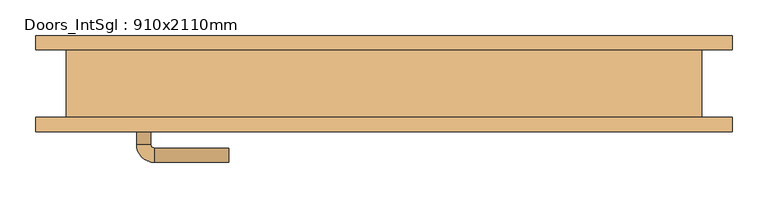
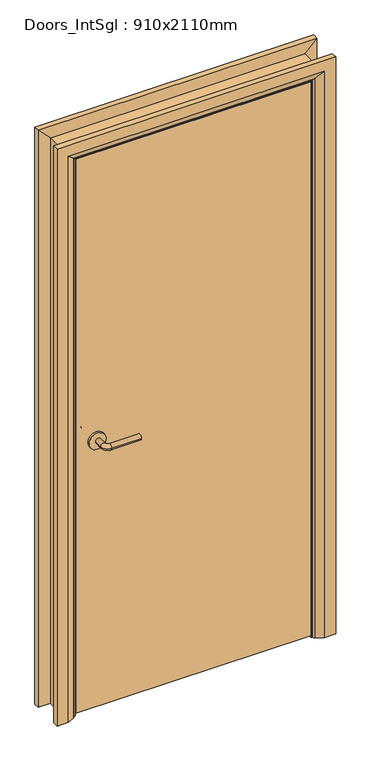
"""IFC4 building model written with IfcOpenShell, lengths in millimetres: door geometry, Doors_IntSgl : 910x2110mm."""

from ifc_helpers import new_model, si_unit, point, frame, frame_2d, origin, place, context, project, spatial, polyline, circle_curve, ellipse_curve, trimmed, segment, composite_curve, outline, extrude, faceted_brep, source, transform, mapped, element, save
from ifc_brep_helpers import plane_surface, cylinder_surface, revolved_surface, advanced_brep


def doors_intsgl_910x2110mm_17b3a64a(model_context):
    return source(origin(), model_context, "Body", "SolidModel", [
        advanced_brep(
        [(-348.0, -1.5, 1000.0), (-328.0, -1.5, 1000.0), (-348.0, 28.5, 1000.0), (-328.0, 28.5, 1000.0), (-323.0, 33.5, 1000.0), (-323.0, 53.5, 1000.0), (-218.0, 53.5, 1000.0), (-218.0, 33.5, 1000.0)],
        [
            (0, 1, circle_curve(frame((-338.0, -1.5, 1000.0), z_axis=(0.0, -1.0, 0.0), x_axis=(1.0, 0.0, 0.0)), 10.0)),
            (1, 0, circle_curve(frame((-338.0, -1.5, 1000.0), z_axis=(0.0, -1.0, 0.0), x_axis=(1.0, 0.0, 0.0)), 10.0)),
            (0, 2),
            (2, 3, circle_curve(frame((-338.0, 28.5, 1000.0), z_axis=(0.0, -1.0, 0.0), x_axis=(1.0, 0.0, 0.0)), 10.0)),
            (3, 1),
            (3, 2, circle_curve(frame((-338.0, 28.5, 1000.0), z_axis=(0.0, -1.0, 0.0), x_axis=(1.0, 0.0, 0.0)), 10.0)),
            (4, 3, circle_curve(frame((-323.0, 28.5, 1000.0), z_axis=(0.0, 0.0, 1.0), x_axis=(-1.0, 0.0, 0.0)), 5.0)),
            (2, 5, circle_curve(frame((-323.0, 28.5, 1000.0), z_axis=(0.0, 0.0, -1.0), x_axis=(-1.0, 0.0, 0.0)), 25.0)),
            (5, 4, circle_curve(frame((-323.0, 43.5, 1000.0), z_axis=(-1.0, 0.0, 0.0), x_axis=(0.0, -1.0, 0.0)), 10.0)),
            (4, 5, circle_curve(frame((-323.0, 43.5, 1000.0), z_axis=(-1.0, 0.0, 0.0), x_axis=(0.0, -1.0, 0.0)), 10.0)),
            (6, 7, circle_curve(frame((-218.0, 43.5, 1000.0), z_axis=(1.0, 0.0, 0.0), x_axis=(0.0, -1.0, 0.0)), 10.0)),
            (7, 6, circle_curve(frame((-218.0, 43.5, 1000.0), z_axis=(1.0, 0.0, 0.0), x_axis=(0.0, -1.0, 0.0)), 10.0)),
            (5, 6),
            (7, 4),
        ],
        [
            plane_surface(frame((-338.0, -1.5, 1000.0), z_axis=(0.0, -1.0, 0.0), x_axis=(0.0, 0.0, 1.0))),
            cylinder_surface(frame((-338.0, -1.5, 1000.0), z_axis=(0.0, -1.0, 0.0), x_axis=(1.0, 0.0, 0.0)), 10.0),
            revolved_surface(trimmed(ellipse_curve(frame((-338.0, 28.5, 1000.0), z_axis=(0.0, -1.0, 0.0), x_axis=(1.0, 0.0, 0.0)), 10.0, 10.0), [point((-348.0, 28.5, 1000.0))], [point((-328.0, 28.5, 1000.0))], True, "CARTESIAN"), (-323.0, 28.5, 1000.0), (0.0, 0.0, -1.0)),
            revolved_surface(trimmed(ellipse_curve(frame((-338.0, 28.5, 1000.0), z_axis=(0.0, -1.0, 0.0), x_axis=(1.0, 0.0, 0.0)), 10.0, 10.0), [point((-328.0, 28.5, 1000.0))], [point((-348.0, 28.5, 1000.0))], True, "CARTESIAN"), (-323.0, 28.5, 1000.0), (0.0, 0.0, -1.0)),
            plane_surface(frame((-218.0, 43.5, 1000.0), z_axis=(1.0, 0.0, 0.0), x_axis=(0.0, 0.0, 1.0))),
            cylinder_surface(frame((-323.0, 43.5, 1000.0), z_axis=(-1.0, 0.0, 0.0), x_axis=(0.0, -1.0, 0.0)), 10.0),
        ],
        [
            (0, [[1, 2]]),
            (1, [[-1, 3, 4, 5]]),
            (1, [[-2, -5, 6, -3]]),
            (2, [[7, -4, 8, 9]]),
            (3, [[-8, -6, -7, 10]]),
            (4, [[11, 12]]),
            (5, [[-9, 13, -12, 14]]),
            (5, [[-10, -14, -11, -13]]),
        ],
    ),
        extrude(outline(composite_curve([segment(trimmed(circle_curve(frame_2d((1000.0, -340.5)), 30.0), [point((1000.0, -370.5))], [point((1000.0, -310.5))], False, "CARTESIAN"), True, "CONTINUOUS"), segment(trimmed(circle_curve(frame_2d((1000.0, -340.5)), 30.0), [point((1000.0, -310.5))], [point((1000.0, -370.5))], False, "CARTESIAN"), True, "CONTINUOUS")], self_intersect=False)), frame((0.0, -9.5, 0.0), z_axis=(0.0, 1.0, 0.0), x_axis=(0.0, 0.0, 1.0)), (0.0, 0.0, 1.0), 8.0),
        advanced_brep(
        [(-348.0, -55.5, 1000.0), (-328.0, -55.5, 1000.0), (-328.0, -85.5, 1000.0), (-348.0, -85.5, 1000.0), (-323.0, -90.5, 1000.0), (-323.0, -110.5, 1000.0), (-218.0, -110.5, 1000.0), (-218.0, -90.5, 1000.0)],
        [
            (0, 1, circle_curve(frame((-338.0, -55.5, 1000.0), z_axis=(0.0, 1.0, 0.0), x_axis=(1.0, 0.0, 0.0)), 10.0)),
            (1, 0, circle_curve(frame((-338.0, -55.5, 1000.0), z_axis=(0.0, 1.0, 0.0), x_axis=(1.0, 0.0, 0.0)), 10.0)),
            (1, 2),
            (2, 3, circle_curve(frame((-338.0, -85.5, 1000.0), z_axis=(0.0, 1.0, 0.0), x_axis=(1.0, 0.0, 0.0)), 10.0)),
            (3, 0),
            (3, 2, circle_curve(frame((-338.0, -85.5, 1000.0), z_axis=(0.0, 1.0, 0.0), x_axis=(1.0, 0.0, 0.0)), 10.0)),
            (4, 5, circle_curve(frame((-323.0, -100.5, 1000.0), z_axis=(-1.0, 0.0, 0.0), x_axis=(0.0, 1.0, 0.0)), 10.0)),
            (5, 3, circle_curve(frame((-323.0, -85.5, 1000.0), z_axis=(0.0, 0.0, -1.0), x_axis=(-1.0, 0.0, 0.0)), 25.0)),
            (2, 4, circle_curve(frame((-323.0, -85.5, 1000.0), z_axis=(0.0, 0.0, 1.0), x_axis=(-1.0, 0.0, 0.0)), 5.0)),
            (5, 4, circle_curve(frame((-323.0, -100.5, 1000.0), z_axis=(-1.0, 0.0, 0.0), x_axis=(0.0, 1.0, 0.0)), 10.0)),
            (6, 7, circle_curve(frame((-218.0, -100.5, 1000.0), z_axis=(1.0, 0.0, 0.0), x_axis=(0.0, 1.0, 0.0)), 10.0)),
            (7, 6, circle_curve(frame((-218.0, -100.5, 1000.0), z_axis=(1.0, 0.0, 0.0), x_axis=(0.0, 1.0, 0.0)), 10.0)),
            (4, 7),
            (6, 5),
        ],
        [
            plane_surface(frame((-338.0, -55.5, 1000.0), z_axis=(0.0, 1.0, 0.0), x_axis=(0.0, 0.0, 1.0))),
            cylinder_surface(frame((-338.0, -55.5, 1000.0), z_axis=(0.0, 1.0, 0.0), x_axis=(1.0, 0.0, 0.0)), 10.0),
            revolved_surface(trimmed(ellipse_curve(frame((-338.0, -85.5, 1000.0), z_axis=(0.0, -1.0, 0.0), x_axis=(1.0, 0.0, 0.0)), 10.0, 10.0), [point((-348.0, -85.5, 1000.0))], [point((-328.0, -85.5, 1000.0))], True, "CARTESIAN"), (-323.0, -85.5, 1000.0), (0.0, 0.0, -1.0)),
            revolved_surface(trimmed(ellipse_curve(frame((-338.0, -85.5, 1000.0), z_axis=(0.0, -1.0, 0.0), x_axis=(1.0, 0.0, 0.0)), 10.0, 10.0), [point((-328.0, -85.5, 1000.0))], [point((-348.0, -85.5, 1000.0))], True, "CARTESIAN"), (-323.0, -85.5, 1000.0), (0.0, 0.0, -1.0)),
            plane_surface(frame((-218.0, -100.5, 1000.0), z_axis=(1.0, 0.0, 0.0), x_axis=(0.0, 0.0, 1.0))),
            cylinder_surface(frame((-323.0, -100.5, 1000.0), z_axis=(-1.0, 0.0, 0.0), x_axis=(0.0, 1.0, 0.0)), 10.0),
        ],
        [
            (0, [[1, 2]]),
            (1, [[3, 4, 5, -2]]),
            (1, [[-5, 6, -3, -1]]),
            (2, [[7, 8, -4, 9]]),
            (3, [[10, -9, -6, -8]]),
            (4, [[11, 12]]),
            (5, [[13, -11, 14, -7]]),
            (5, [[-14, -12, -13, -10]]),
        ],
    ),
        extrude(outline(composite_curve([segment(trimmed(circle_curve(frame_2d((1000.0, -340.5)), 30.0), [point((1000.0, -370.5))], [point((1000.0, -310.5))], False, "CARTESIAN"), True, "CONTINUOUS"), segment(trimmed(circle_curve(frame_2d((1000.0, -340.5)), 30.0), [point((1000.0, -310.5))], [point((1000.0, -370.5))], False, "CARTESIAN"), True, "CONTINUOUS")], self_intersect=False)), frame((0.0, -55.5, 0.0), z_axis=(0.0, 1.0, 0.0), x_axis=(0.0, 0.0, 1.0)), (0.0, 0.0, 1.0), 8.0),
        extrude(outline(polyline([(413.0, -9.5), (413.0, -47.5), (-413.0, -47.5), (-413.0, -9.5), (413.0, -9.5)])), frame((0.0, 0.0, 8.0), z_axis=(0.0, 0.0, 1.0), x_axis=(1.0, 0.0, 0.0)), (0.0, 0.0, 1.0), 2060.0),
        advanced_brep(
        [(490.0, -67.5, 0.0), (450.0, -67.5, 0.0), (424.0, -53.5, 0.0), (420.0, -47.5, 0.0), (490.0, -47.5, 0.0), (490.0, -47.5, 2145.0), (490.0, -67.5, 2145.0), (420.0, -47.5, 2075.0), (-420.0, -47.5, 2075.0), (-420.0, -47.5, 0.0), (-490.0, -47.5, 0.0), (-490.0, -47.5, 2145.0), (424.0, -53.5, 2079.0), (450.0, -67.5, 2105.0), (-490.0, -67.5, 2145.0), (-490.0, -67.5, 0.0), (-450.0, -67.5, 0.0), (-450.0, -67.5, 2105.0), (-424.0, -53.5, 2079.0), (-424.0, -53.5, 0.0)],
        [
            (0, 1),
            (1, 2),
            (2, 3, circle_curve(frame((428.0, -46.5, 0.0), z_axis=(0.0, 0.0, -1.0), x_axis=(1.0, 0.0, 0.0)), 8.0622577)),
            (3, 4),
            (4, 0),
            (4, 5),
            (5, 6),
            (6, 0),
            (3, 7),
            (7, 8),
            (8, 9),
            (9, 10),
            (10, 11),
            (11, 5),
            (2, 12),
            (12, 7, ellipse_curve(frame((428.0, -46.5, 2083.0), z_axis=(0.7071067811865475, 0.0, -0.7071067811865475), x_axis=(-0.7071067811865474, 0.0, -0.7071067811865476)), 11.4017543, 8.0622577)),
            (1, 13),
            (13, 12),
            (6, 14),
            (14, 15),
            (15, 16),
            (16, 17),
            (17, 13),
            (11, 14),
            (12, 18),
            (18, 8, ellipse_curve(frame((-428.0, -46.5, 2083.0), z_axis=(0.7071067811865475, 0.0, 0.7071067811865475), x_axis=(0.7071067811865476, 0.0, -0.7071067811865474)), 11.4017543, 8.0622577)),
            (17, 18),
            (15, 10),
            (9, 19, circle_curve(frame((-428.0, -46.5, 0.0), z_axis=(0.0, 0.0, -1.0), x_axis=(-1.0, 0.0, 0.0)), 8.0622577)),
            (19, 16),
            (18, 19),
        ],
        [
            plane_surface(frame((420.0, -47.5, 0.0), z_axis=(0.0, 0.0, -1.0), x_axis=(0.0, 1.0, 0.0))),
            plane_surface(frame((490.0, -67.5, 0.0), z_axis=(1.0, 0.0, 0.0), x_axis=(0.0, 0.0, 1.0))),
            plane_surface(frame((490.0, -47.5, 0.0), z_axis=(0.0, 1.0, 0.0), x_axis=(0.0, 0.0, 1.0))),
            cylinder_surface(frame((428.0, -46.5, 0.0), z_axis=(0.0, 0.0, -1.0), x_axis=(1.0, 0.0, 0.0)), 8.0622577),
            plane_surface(frame((424.0, -53.5, 0.0), z_axis=(-0.4740998230350126, -0.880471099922178, 0.0), x_axis=(0.0, 0.0, 1.0))),
            plane_surface(frame((450.0, -67.5, 0.0), z_axis=(0.0, -1.0, 0.0), x_axis=(0.0, 0.0, 1.0))),
            plane_surface(frame((490.0, -67.5, 2145.0), z_axis=(0.0, 0.0, 1.0), x_axis=(-1.0, 0.0, 0.0))),
            cylinder_surface(frame((420.0, -46.5, 2083.0), z_axis=(1.0, 0.0, 0.0), x_axis=(0.0, 0.0, 1.0)), 8.0622577),
            plane_surface(frame((424.0, -53.5, 2079.0), z_axis=(0.0, -0.8804710999221764, -0.4740998230350154), x_axis=(-1.0, 0.0, 0.0))),
            plane_surface(frame((-420.0, -47.5, 0.0), z_axis=(0.0, 0.0, -1.0), x_axis=(0.0, 1.0, 0.0))),
            plane_surface(frame((-490.0, -67.5, 2145.0), z_axis=(-1.0, 0.0, 0.0), x_axis=(0.0, 0.0, -1.0))),
            cylinder_surface(frame((-428.0, -46.5, 2075.0), z_axis=(0.0, 0.0, 1.0), x_axis=(-1.0, 0.0, 0.0)), 8.0622577),
            plane_surface(frame((-424.0, -53.5, 2079.0), z_axis=(0.47409982303501824, -0.8804710999221749, 0.0), x_axis=(0.0, 0.0, -1.0))),
        ],
        [
            (0, [[1, 2, 3, 4, 5]]),
            (1, [[6, 7, 8, -5]]),
            (2, [[9, 10, 11, 12, 13, 14, -6, -4]]),
            (3, [[15, 16, -9, -3]]),
            (4, [[17, 18, -15, -2]]),
            (5, [[-8, 19, 20, 21, 22, 23, -17, -1]]),
            (6, [[-14, 24, -19, -7]]),
            (7, [[25, 26, -10, -16]]),
            (8, [[-23, 27, -25, -18]]),
            (9, [[28, -12, 29, 30, -21]]),
            (10, [[-13, -28, -20, -24]]),
            (11, [[31, -29, -11, -26]]),
            (12, [[-22, -30, -31, -27]]),
        ],
    ),
        extrude(outline(polyline([(0.0, -396.0), (2051.0, -396.0), (2051.0, 396.0), (0.0, 396.0), (0.0, 415.0), (2070.0, 415.0), (2070.0, -415.0), (0.0, -415.0), (0.0, -396.0)])), frame((0.0, -7.5, 0.0), z_axis=(0.0, 1.0, 0.0), x_axis=(0.0, 0.0, 1.0)), (0.0, 0.0, 1.0), 32.0),
        advanced_brep(
        [(-490.0, 67.5, 0.0), (-450.0, 67.5, 0.0), (-424.0, 53.5, 0.0), (-420.0, 47.5, 0.0), (-490.0, 47.5, 0.0), (-490.0, 47.5, 2145.0), (-490.0, 67.5, 2145.0), (-420.0, 47.5, 2075.0), (-424.0, 53.5, 2079.0), (-450.0, 67.5, 2105.0), (490.0, 47.5, 2145.0), (490.0, 67.5, 2145.0), (420.0, 47.5, 2075.0), (424.0, 53.5, 2079.0), (450.0, 67.5, 2105.0), (490.0, 67.5, 0.0), (490.0, 47.5, 0.0), (420.0, 47.5, 0.0), (424.0, 53.5, 0.0), (450.0, 67.5, 0.0)],
        [
            (0, 1),
            (1, 2),
            (2, 3, circle_curve(frame((-428.0, 46.5, 0.0), z_axis=(0.0, 0.0, -1.0), x_axis=(-1.0, 0.0, 0.0)), 8.0622577)),
            (3, 4),
            (4, 0),
            (4, 5),
            (5, 6),
            (6, 0),
            (3, 7),
            (7, 5),
            (2, 8),
            (8, 7, ellipse_curve(frame((-428.0, 46.5, 2083.0), z_axis=(-0.7071067811865475, 0.0, -0.7071067811865475), x_axis=(0.7071067811865474, 0.0, -0.7071067811865476)), 11.4017543, 8.0622577)),
            (1, 9),
            (9, 8),
            (6, 9),
            (5, 10),
            (10, 11),
            (11, 6),
            (7, 12),
            (12, 10),
            (8, 13),
            (13, 12, ellipse_curve(frame((428.0, 46.5, 2083.0), z_axis=(-0.7071067811865475, 0.0, 0.7071067811865475), x_axis=(-0.7071067811865476, 0.0, -0.7071067811865474)), 11.4017543, 8.0622577)),
            (9, 14),
            (14, 13),
            (11, 14),
            (15, 16),
            (16, 17),
            (17, 18, circle_curve(frame((428.0, 46.5, 0.0), z_axis=(0.0, 0.0, -1.0), x_axis=(1.0, 0.0, 0.0)), 8.0622577)),
            (18, 19),
            (19, 15),
            (10, 16),
            (15, 11),
            (12, 17),
            (13, 18),
            (14, 19),
        ],
        [
            plane_surface(frame((-420.0, 120.3010989, 0.0), z_axis=(0.0, 0.0, -1.0), x_axis=(1.0, 0.0, 0.0))),
            plane_surface(frame((-490.0, 67.5, 0.0), z_axis=(-1.0, 0.0, 0.0), x_axis=(0.0, 0.0, 1.0))),
            plane_surface(frame((-490.0, 47.5, 0.0), z_axis=(0.0, -1.0, 0.0), x_axis=(0.0, 0.0, 1.0))),
            cylinder_surface(frame((-428.0, 46.5, 0.0), z_axis=(0.0, 0.0, -1.0), x_axis=(-1.0, 0.0, 0.0)), 8.0622577),
            plane_surface(frame((-424.0, 53.5, 0.0), z_axis=(0.4740998230350183, 0.8804710999221749, 0.0), x_axis=(0.0, 0.0, 1.0))),
            plane_surface(frame((-450.0, 67.5, 0.0), z_axis=(0.0, 1.0, 0.0), x_axis=(0.0, 0.0, 1.0))),
            plane_surface(frame((-490.0, 67.5, 2145.0), z_axis=(0.0, 0.0, 1.0), x_axis=(1.0, 0.0, 0.0))),
            plane_surface(frame((-490.0, 47.5, 2145.0), z_axis=(0.0, -1.0, 0.0), x_axis=(1.0, 0.0, 0.0))),
            cylinder_surface(frame((-420.0, 46.5, 2083.0), z_axis=(-1.0, 0.0, 0.0), x_axis=(0.0, 0.0, 1.0)), 8.0622577),
            plane_surface(frame((-424.0, 53.5, 2079.0), z_axis=(0.0, 0.8804710999221749, -0.4740998230350183), x_axis=(1.0, 0.0, 0.0))),
            plane_surface(frame((-450.0, 67.5, 2105.0), z_axis=(0.0, 1.0, 0.0), x_axis=(1.0, 0.0, 0.0))),
            plane_surface(frame((420.0, 120.3010989, 0.0), z_axis=(0.0, 0.0, -1.0), x_axis=(-1.0, 0.0, 0.0))),
            plane_surface(frame((490.0, 67.5, 2145.0), z_axis=(1.0, 0.0, 0.0), x_axis=(0.0, 0.0, -1.0))),
            plane_surface(frame((490.0, 47.5, 2145.0), z_axis=(0.0, -1.0, 0.0), x_axis=(0.0, 0.0, -1.0))),
            cylinder_surface(frame((428.0, 46.5, 2075.0), z_axis=(0.0, 0.0, 1.0), x_axis=(1.0, 0.0, 0.0)), 8.0622577),
            plane_surface(frame((424.0, 53.5, 2079.0), z_axis=(-0.4740998230350183, 0.8804710999221749, 0.0), x_axis=(0.0, 0.0, -1.0))),
            plane_surface(frame((450.0, 67.5, 2105.0), z_axis=(0.0, 1.0, 0.0), x_axis=(0.0, 0.0, -1.0))),
        ],
        [
            (0, [[1, 2, 3, 4, 5]]),
            (1, [[6, 7, 8, -5]]),
            (2, [[9, 10, -6, -4]]),
            (3, [[11, 12, -9, -3]]),
            (4, [[13, 14, -11, -2]]),
            (5, [[-8, 15, -13, -1]]),
            (6, [[16, 17, 18, -7]]),
            (7, [[19, 20, -16, -10]]),
            (8, [[21, 22, -19, -12]]),
            (9, [[23, 24, -21, -14]]),
            (10, [[-18, 25, -23, -15]]),
            (11, [[26, 27, 28, 29, 30]]),
            (12, [[31, -26, 32, -17]]),
            (13, [[33, -27, -31, -20]]),
            (14, [[34, -28, -33, -22]]),
            (15, [[35, -29, -34, -24]]),
            (16, [[-32, -30, -35, -25]]),
        ],
    ),
        faceted_brep([(-415.0, -47.5, 0.0), (-447.0, -47.5, 0.0), (-447.0, 47.5, 0.0), (-415.0, 47.5, 0.0), (-415.0, 47.5, 2070.0), (-415.0, -47.5, 2070.0), (-447.0, 47.5, 2102.0), (-447.0, -47.5, 2102.0), (415.0, 47.5, 2070.0), (415.0, -47.5, 2070.0), (447.0, 47.5, 2102.0), (447.0, -47.5, 2102.0), (415.0, -47.5, 0.0), (415.0, 47.5, 0.0), (447.0, 47.5, 0.0), (447.0, -47.5, 0.0)], [[[0, 1, 2, 3]], [[3, 4, 5, 0]], [[2, 6, 4, 3]], [[1, 7, 6, 2]], [[0, 5, 7, 1]], [[4, 8, 9, 5]], [[6, 10, 8, 4]], [[7, 11, 10, 6]], [[5, 9, 11, 7]], [[12, 13, 14, 15]], [[8, 13, 12, 9]], [[10, 14, 13, 8]], [[11, 15, 14, 10]], [[9, 12, 15, 11]]]),
    ])


if __name__ == "__main__":
    model = new_model("IFC4")
    model_context = context("Model", 3, world=origin())
    ifc_project = project(units=[si_unit("LENGTHUNIT", "METRE", prefix="MILLI")], contexts=[model_context])
    site = spatial("IfcSite", under=ifc_project)
    building = spatial("IfcBuilding", under=site)
    placement = place(None, origin())
    doors_intsgl_910x2110mm_shape = doors_intsgl_910x2110mm_17b3a64a(model_context)
    element("IfcDoor", 1, ObjectType="Doors_IntSgl : 910x2110mm", at=placement, inside=building, context=model_context, shape_type="MappedRepresentation", body=[
        mapped(doors_intsgl_910x2110mm_shape, transform((0.0, 0.0, 0.0), x_axis=(1.0, 0.0, 0.0), y_axis=(0.0, 1.0, 0.0), z_axis=(0.0, 0.0, 1.0))),
    ])
    save(model, "model.ifc")

# Revit data of these elements
# Type "Doors_IntSgl : 910x2110mm"
#   Construction Type Id = "MDOOR"
#   Type Mark = "41"
#   Type Comments = "Internal Single"
#   Operation = "SingleSwingRight"
#   Manufacturer = "Revit"
#   Keynote = "L20"
#   Description = "Internal Single Door"
#   Analytic Construction = "Metal"
#   UnderCut = 8 mm
#   Tolerance = 2 mm
#   Thickness = 38 mm
#   Thermal Resistance (R) = 0.270117 (m²·K)/W
#   Structural Tolerance = 8 mm
#   StopDepth = 32 mm
#   Stop Thickness = 19 mm
#   Rough Width = 910 mm
#   Rough Height = 2110 mm
#   Height to Top Lock Rail = 1000 mm
#   Heat Transfer Coefficient (U) = 3.7021 W/(m²·K)
#   Handle Z Distance = 1000 mm
#   Handle X Distance = 75 mm
#   Frame Thickness = 32 mm
#   Door Panel Width = 826 mm
#   Door Panel Thickness = 38 mm
#   Door Panel Offset = 0 mm
#   Height = 2110 mm
#   Width = 910 mm
#   Door Panel Height = 2060 mm
#   Architrave Setback = 5 mm
#   Vis - Ironmongery = yes
#   Material Ironmongery = Door - Handle
#   Material Frame = Door - Frame/Mullion (1)
#   Material Door = Door - Panel
#   Material Architrave = Door - Architrave
#   Visual Light Transmittance = 0
#   Solar Heat Gain Coefficient = 0
#   Function = (empty or 0)
#   Wall Closure = (empty or 0)
# Element 1 (IfcDoor, "Doors_IntSgl : 910x2110mm")
#   Materials on its faces: "Door - Architrave", "Door - Handle", "Door - Frame/Mullion (1)", "Door - Panel"
# Materials
#   "Door - Handle": class "Miscellaneous", colour RGB 0 0 0, transparency 0, Keynote = "P21"
#   "Door - Frame/Mullion (1)": class "Wood", colour RGB 212 179 113, transparency 0, Keynote = "L20", Cost = 0
#   "Door - Panel": class "Wood", colour RGB 210 159 95, transparency 0, Keynote = "L20"
#   "Door - Architrave": class "Wood", colour RGB 154 90 5, transparency 0, Keynote = "P20"
